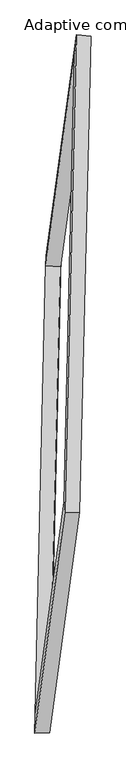
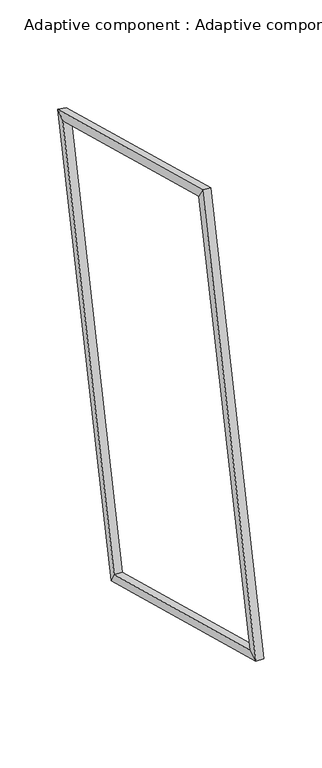
"""IFC4 building model written with IfcOpenShell, lengths in millimetres: proxy geometry, Adaptive component : Adaptive component."""

from ifc_helpers import new_model, si_unit, origin, place, context, project, spatial, faceted_brep, source, transform, mapped, element, save


def adaptive_component_adaptive_component_a8c90d70(model_context):
    return source(origin(), model_context, "Body", "Brep", [
        faceted_brep([(64.3764682, 1035.4277638, 2679.5342557), (129.0457399, 1029.4199143, 2675.4589597), (81.4425051, -938.6466846, 3245.6517004), (16.6276889, -938.6561049, 3251.4703335), (71.4690839, 1115.6674492, 2723.7097094), (20.704416, -983.1026857, 3331.7701764), (136.1383556, 1109.6595997, 2719.6344134), (85.5192322, -983.0932654, 3325.9515433), (-45.8434374, -1872.0425655, 13.3333143), (-110.8951633, -1873.7892594, 13.1358276), (-111.7275367, -1954.2345851, -31.2267664), (-46.6758107, -1952.4878912, -31.0292797), (1.7597974, 96.0240334, -556.8594264), (-63.1463839, 100.2946093, -558.8002502), (-60.9628687, 144.5355497, -639.2872334), (3.9433126, 140.2649739, -637.3464096)], [[[0, 1, 2, 3]], [[4, 0, 3, 5]], [[6, 4, 5, 7]], [[1, 6, 7, 2]], [[3, 2, 8, 9]], [[5, 3, 9, 10]], [[7, 5, 10, 11]], [[2, 7, 11, 8]], [[9, 8, 12, 13]], [[10, 9, 13, 14]], [[11, 10, 14, 15]], [[8, 11, 15, 12]], [[13, 12, 1, 0]], [[14, 13, 0, 4]], [[15, 14, 4, 6]], [[12, 15, 6, 1]]]),
    ])


if __name__ == "__main__":
    model = new_model("IFC4")
    model_context = context("Model", 3, world=origin())
    ifc_project = project(units=[si_unit("LENGTHUNIT", "METRE", prefix="MILLI")], contexts=[model_context])
    site = spatial("IfcSite", under=ifc_project)
    building = spatial("IfcBuilding", under=site)
    placement = place(None, origin())
    adaptive_component_adaptive_component_shape = adaptive_component_adaptive_component_a8c90d70(model_context)
    element("IfcBuildingElementProxy", 1, Name="Adaptive component : Adaptive component", ObjectType="Adaptive component : Adaptive component", at=placement, inside=building, context=model_context, shape_type="MappedRepresentation", body=[
        mapped(adaptive_component_adaptive_component_shape, transform((0.0, 0.0, 0.0), x_axis=(1.0, 0.0, 0.0), y_axis=(0.0, 1.0, 0.0), z_axis=(0.0, 0.0, 1.0))),
    ])
    save(model, "model.ifc")

# Revit data of these elements
# Type "Adaptive component : Adaptive component"
#   r [instance default] = 2063.125 mm
#   2r [instance default] = 4126.251 mm
#   Number [instance default] = 5
#   Default Elevation = 0
# Element 1 (IfcBuildingElementProxy, "Adaptive component : Adaptive component")
#   r = 2062.428 mm
#   2r = 4124.856 mm
#   Number = 4
